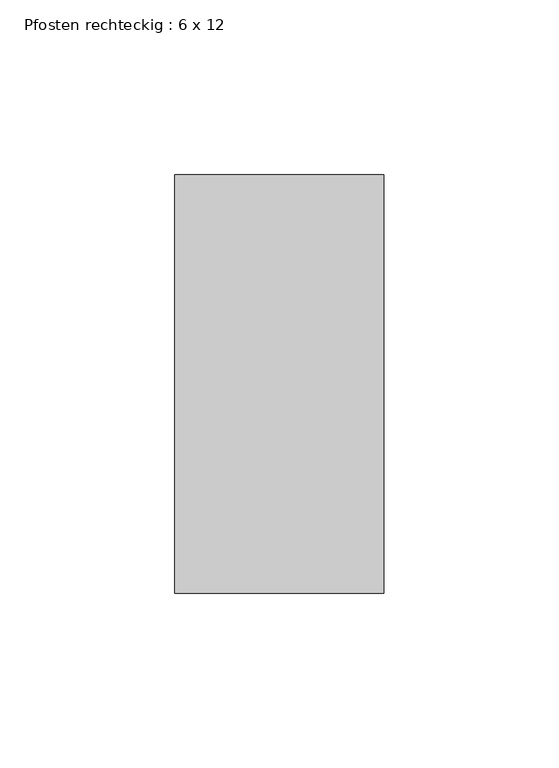
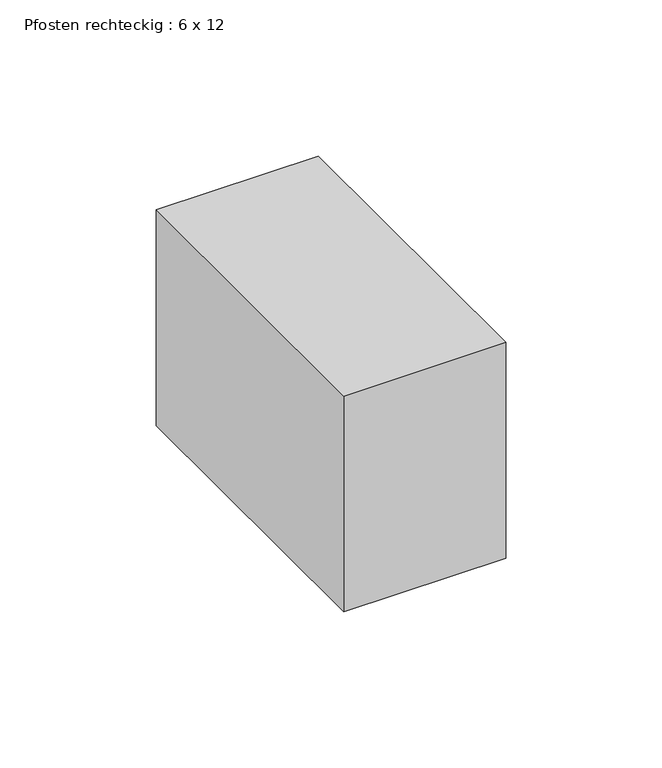
"""IFC4 building model written with IfcOpenShell, lengths in millimetres: member geometry, Pfosten rechteckig : 6 x 12."""

from ifc_helpers import new_model, si_unit, frame, origin, place, context, project, spatial, polyline, outline, extrude, source, transform, mapped, element, save


def pfosten_rechteckig_6_x_12_6cbda8fd(model_context):
    return source(origin(), model_context, "Body", "SweptSolid", [
        extrude(outline(polyline([(0.0, 60.0), (0.0, -60.0), (-60.0, -60.0), (-60.0, 60.0), (0.0, 60.0)])), frame((0.0, 0.0, -84.3558419), z_axis=(0.0, 0.0, 1.0), x_axis=(1.0, 0.0, 0.0)), (0.0, 0.0, 1.0), 84.3558419),
    ])


if __name__ == "__main__":
    model = new_model("IFC4")
    model_context = context("Model", 3, world=origin())
    ifc_project = project(units=[si_unit("LENGTHUNIT", "METRE", prefix="MILLI")], contexts=[model_context])
    site = spatial("IfcSite", under=ifc_project)
    building = spatial("IfcBuilding", under=site)
    placement = place(None, origin())
    pfosten_rechteckig_6_x_12_shape = pfosten_rechteckig_6_x_12_6cbda8fd(model_context)
    element("IfcMember", 1, ObjectType="Pfosten rechteckig : 6 x 12", at=placement, inside=building, context=model_context, shape_type="MappedRepresentation", body=[
        mapped(pfosten_rechteckig_6_x_12_shape, transform((0.0, 0.0, 0.0), x_axis=(1.0, 0.0, 0.0), y_axis=(0.0, 1.0, 0.0), z_axis=(0.0, 0.0, 1.0))),
    ])
    save(model, "model.ifc")

# Revit data of these elements
# Type "Pfosten rechteckig : 6 x 12"
#   built-in parameter 1007304 = 0.393701 (stored number, unit not read)
#   built-in parameter 1007301 = 0.0984252 (stored number, unit not read)
#   built-in parameter 1007300 = 0.0984252 (stored number, unit not read)
# Element 1 (IfcMember, "Pfosten rechteckig : 6 x 12")
#   Materials on its faces: "Metall - verzinkt"
# Materials
#   "Metall - verzinkt": class "Allgemeines", colour RGB 200 200 200, transparency 0, Cost = 0
